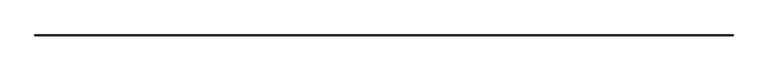
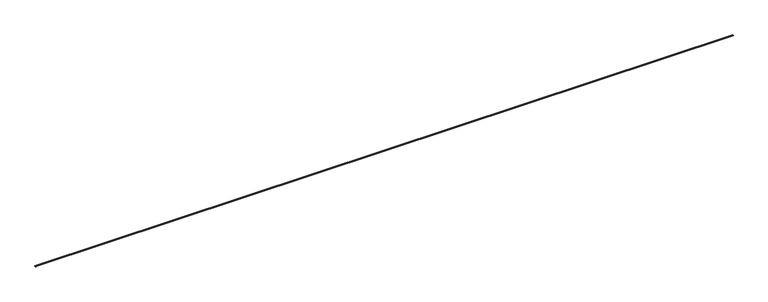
"""IFC4 building model written with IfcOpenShell, lengths in millimetres: proxy geometry, Generic Models 3:Generic Models 1:4:Generic Models 1:4 : Generic Models 3:Generic Models 1:300625:1:Generic Models 1:4:Generic Models 1:4 : Generic Models 3:Generic Models 1:300625:1 : Generic Models 3:Generic Models 1:4:Generic Models 1:4 : Generic Models 3:Generic Models 1:300625:338780:2 : Generic Models 3:Generic Models 1:4:Generic Models 1:4 : Generic Models 3:Generic Models 1:300625:1:Generic Models 1:4:Generic Models 1:4 : Generic Models 3:Generic Models 1:300625:1 : Generic Models 3:Generic Models 1:4:Generic Models 1:4 : Generic Models 3:Generic Models 1:300625:338780:317135."""

import ifcopenshell
import ifcopenshell.guid

model = None  # the IFC model being written
_history = None  # IfcOwnerHistory: only IFC2X3 demands one
_inside = {}  # id of a spatial element -> (the spatial element, [elements in it])
_under = {}  # id of a project, library or spatial element -> (it, [spatial elements below it])
_declared = {}  # id of a project -> (the project, [libraries it declares])
_typed = {}  # id of a type object -> (the type object, [elements of that type])
_made_of = {}  # id of a material, layer set ... -> (it, [elements and type objects made of it])


def new_model(schema):
    """Start an empty IFC model of exactly this schema.

    Asked for "IFC4X3", IfcOpenShell would pick the latest addendum, in which some entities
    have other attributes; the version numbers below select the first issue.
    IFC2X3 requires an IfcOwnerHistory on every rooted entity: one is made here for all.
    """
    global model, _history
    if schema == "IFC4X3":
        model = ifcopenshell.file(schema_version=(4, 3, 0, 0))
    else:
        model = ifcopenshell.file(schema=schema)
    _inside.clear()
    _under.clear()
    _declared.clear()
    _typed.clear()
    _made_of.clear()
    _history = None
    if model.schema == "IFC2X3":
        org = make("IfcOrganization", Name="unknown")
        user = make(
            "IfcPersonAndOrganization",
            ThePerson=make("IfcPerson", FamilyName="unknown"),
            TheOrganization=org,
        )
        app = make(
            "IfcApplication",
            ApplicationDeveloper=org,
            Version="unknown",
            ApplicationFullName="unknown",
            ApplicationIdentifier="unknown",
        )
        _history = make(
            "IfcOwnerHistory",
            OwningUser=user,
            OwningApplication=app,
            ChangeAction="ADDED",
            CreationDate=0,
        )
    return model


def make(cls, **values):
    """One entity of the class cls with the attributes given. An attribute that is None is left unset."""
    return model.create_entity(
        cls, **{name: value for name, value in values.items() if value is not None}
    )


def rooted(cls, **values):
    """An entity with a GlobalId (a new one), such as an element, a storey or a relation."""
    return make(cls, GlobalId=ifcopenshell.guid.new(), OwnerHistory=_history, **values)


def si_unit(unit_type, name, prefix=None):
    """IfcSIUnit, for example si_unit("LENGTHUNIT", "METRE", prefix="MILLI")."""
    return make("IfcSIUnit", UnitType=unit_type, Prefix=prefix, Name=name)


def assignment(units):
    """IfcUnitAssignment: the units of a project."""
    return None if units is None else make("IfcUnitAssignment", Units=units)


def point(xyz):
    """IfcCartesianPoint."""
    return None if xyz is None else make("IfcCartesianPoint", Coordinates=xyz)


def direction(xyz):
    """IfcDirection."""
    return None if xyz is None else make("IfcDirection", DirectionRatios=xyz)


def frame(location, z_axis=None, x_axis=None):
    """IfcAxis2Placement3D, a coordinate frame: its origin and axes. An axis left out is left unset."""
    return make(
        "IfcAxis2Placement3D",
        Location=point(location),
        Axis=direction(z_axis),
        RefDirection=direction(x_axis),
    )


def origin():
    """The frame at (0, 0, 0) with its axes left unset."""
    return frame((0.0, 0.0, 0.0))


def place(relative_to, where):
    """IfcLocalPlacement: puts the frame where relative to a parent placement (None: the world)."""
    return make(
        "IfcLocalPlacement", PlacementRelTo=relative_to, RelativePlacement=where
    )


def context(
    kind, dimensions, precision=None, world=None, true_north=None, identifier=None
):
    """IfcGeometricRepresentationContext, for example the 3D "Model" context."""
    return make(
        "IfcGeometricRepresentationContext",
        ContextIdentifier=identifier,
        ContextType=kind,
        CoordinateSpaceDimension=dimensions,
        Precision=precision,
        WorldCoordinateSystem=world,
        TrueNorth=true_north,
    )


def project(units=None, contexts=None):
    """IfcProject with its units and contexts."""
    return rooted(
        "IfcProject",
        Name="project",
        RepresentationContexts=contexts,
        UnitsInContext=assignment(units),
    )


def spatial(cls, under=None, at=None, **own):
    """A site, building, storey or space (cls), placed at a placement, below another one or the project."""
    s = rooted(cls, ObjectPlacement=at, **own)
    if under is not None:
        _under.setdefault(under.id(), (under, []))[1].append(s)
    return s


def polyline(points):
    """IfcPolyline through the points."""
    return make("IfcPolyline", Points=[point(p) for p in points])


def outline(outer, holes=None, kind="AREA"):
    """IfcArbitraryClosedProfileDef: a profile drawn as a closed curve; with holes, ...WithVoids."""
    if holes is None:
        return make("IfcArbitraryClosedProfileDef", ProfileType=kind, OuterCurve=outer)
    return make(
        "IfcArbitraryProfileDefWithVoids",
        ProfileType=kind,
        OuterCurve=outer,
        InnerCurves=holes,
    )


def extrude(swept, where, along, depth):
    """IfcExtrudedAreaSolid: the profile swept, set in the frame where, extruded along a direction by depth."""
    return make(
        "IfcExtrudedAreaSolid",
        SweptArea=swept,
        Position=where,
        ExtrudedDirection=direction(along),
        Depth=depth,
    )


def shape(context_of_items, identifier, shape_type, items):
    """IfcShapeRepresentation: the items that make up one representation, for example the "Body"."""
    return make(
        "IfcShapeRepresentation",
        ContextOfItems=context_of_items,
        RepresentationIdentifier=identifier,
        RepresentationType=shape_type,
        Items=items,
    )


def source(mapping_origin, context_of_items, identifier, shape_type, items):
    """IfcRepresentationMap: a shape defined once, which mapped items show again and again."""
    return make(
        "IfcRepresentationMap",
        MappingOrigin=mapping_origin,
        MappedRepresentation=shape(context_of_items, identifier, shape_type, items),
    )


def transform(
    local_origin,
    x_axis=None,
    y_axis=None,
    z_axis=None,
    scale=None,
    scale2=None,
    scale3=None,
    uniform=True,
):
    """IfcCartesianTransformationOperator3D, or its non-uniform kind. x_axis, y_axis, z_axis: its Axis1, 2, 3."""
    if uniform:
        return make(
            "IfcCartesianTransformationOperator3D",
            Axis1=direction(x_axis),
            Axis2=direction(y_axis),
            LocalOrigin=point(local_origin),
            Scale=scale,
            Axis3=direction(z_axis),
        )
    return make(
        "IfcCartesianTransformationOperator3DnonUniform",
        Axis1=direction(x_axis),
        Axis2=direction(y_axis),
        LocalOrigin=point(local_origin),
        Scale=scale,
        Axis3=direction(z_axis),
        Scale2=scale2,
        Scale3=scale3,
    )


def mapped(mapping_source, mapping_target):
    """IfcMappedItem: shows the shape of a source again, moved by a transform."""
    return make(
        "IfcMappedItem", MappingSource=mapping_source, MappingTarget=mapping_target
    )


def made_of(thing, what):
    """Note that an element or type object is made of a material, layer set ...; save() writes the relation."""
    if what is not None:
        _made_of.setdefault(what.id(), (what, []))[1].append(thing)
    return thing


def element(
    cls,
    number,
    at=None,
    inside=None,
    cuts=None,
    type_object=None,
    material=None,
    context=None,
    identifier="Body",
    shape_type=None,
    held_by="IfcProductDefinitionShape",
    body=None,
    shapes=None,
    **own,
):
    """One element of the class cls, such as IfcWall. Its Tag is "e" and its number.

    at: its placement. inside: the storey or other place that contains it. cuts: it is an
    opening in that element (IfcRelVoidsElement). A single representation is given by context,
    identifier, shape_type and body (its items); several are given by shapes. held_by: the class
    of the entity that holds the representations. save() writes the other relations.
    """
    e = rooted(cls, Tag="e%d" % number, ObjectPlacement=at, **own)
    if body is not None:
        shapes = [shape(context, identifier, shape_type, body)]
    if shapes is not None:
        e.Representation = make(held_by, Representations=shapes)
    if inside is not None:
        _inside.setdefault(inside.id(), (inside, []))[1].append(e)
    if cuts is not None:
        rooted(
            "IfcRelVoidsElement", RelatingBuildingElement=cuts, RelatedOpeningElement=e
        )
    if type_object is not None:
        _typed.setdefault(type_object.id(), (type_object, []))[1].append(e)
    return made_of(e, material)


def aggregate(whole, parts):
    """IfcRelAggregates: a whole, such as a stair, and the parts it consists of."""
    return rooted("IfcRelAggregates", RelatingObject=whole, RelatedObjects=parts)


def save(model, path):
    """Write the relations noted so far, then the file.

    IfcRelAggregates (storeys below a building ...), IfcRelContainedInSpatialStructure (elements
    in a storey), IfcRelDefinesByType, IfcRelAssociatesMaterial and IfcRelDeclares: one each for
    every whole, place, type object, material and project.
    """
    for whole, parts in _under.values():
        aggregate(whole, parts)
    for where, things in _inside.values():
        rooted(
            "IfcRelContainedInSpatialStructure",
            RelatedElements=things,
            RelatingStructure=where,
        )
    for kind, things in _typed.values():
        rooted("IfcRelDefinesByType", RelatedObjects=things, RelatingType=kind)
    for what, things in _made_of.values():
        rooted("IfcRelAssociatesMaterial", RelatedObjects=things, RelatingMaterial=what)
    for by, libraries in _declared.values():
        rooted("IfcRelDeclares", RelatingContext=by, RelatedDefinitions=libraries)
    model.write(path)


def generic_models_aa0125ff(model_context):
    return source(origin(), model_context, "Body", "SweptSolid", [
        extrude(outline(polyline([(-579088.4739295, 3713.8232545), (-579094.6612723, 3713.8232545), (-579094.1146795, 3714.4746585), (-579093.8638533, 3715.4107545), (-579094.1146795, 3716.3468505), (-579094.6612723, 3716.9982545), (-579088.4739295, 3716.9982545), (-579089.0205223, 3716.3468505), (-579089.2713485, 3715.4107545), (-579089.0205223, 3714.4746585), (-579088.4739295, 3713.8232545)])), frame((591306.0367239, 0.0, 0.0), z_axis=(1.0, 0.0, 0.0), x_axis=(0.0, 1.0, 0.0)), (0.0, 0.0, 1.0), 4876.8),
    ])


if __name__ == "__main__":
    model = new_model("IFC4")
    model_context = context("Model", 3, world=origin())
    ifc_project = project(units=[si_unit("LENGTHUNIT", "METRE", prefix="MILLI")], contexts=[model_context])
    site = spatial("IfcSite", under=ifc_project)
    building = spatial("IfcBuilding", under=site)
    placement = place(None, origin())
    generic_models_shape = generic_models_aa0125ff(model_context)
    element("IfcBuildingElementProxy", 1, Name="Generic Models 3:Generic Models 1:4:Generic Models 1:4 : Generic Models 3:Generic Models 1:300625:1:Generic Models 1:4:Generic Models 1:4 : Generic Models 3:Generic Models 1:300625:1 : Generic Models 3:Generic Models 1:4:Generic Models 1:4 : Generic Models 3:Generic Models 1:300625:338780:2 : Generic Models 3:Generic Models 1:4:Generic Models 1:4 : Generic Models 3:Generic Models 1:300625:1:Generic Models 1:4:Generic Models 1:4 : Generic Models 3:Generic Models 1:300625:1 : Generic Models 3:Generic Models 1:4:Generic Models 1:4 : Generic Models 3:Generic Models 1:300625:338780:317135", ObjectType="Generic Models 3:Generic Models 1:4:Generic Models 1:4 : Generic Models 3:Generic Models 1:300625:1:Generic Models 1:4:Generic Models 1:4 : Generic Models 3:Generic Models 1:300625:1 : Generic Models 3:Generic Models 1:4:Generic Models 1:4 : Generic Models 3:Generic Models 1:300625:338780:2 : Generic Models 3:Generic Models 1:4:Generic Models 1:4 : Generic Models 3:Generic Models 1:300625:1:Generic Models 1:4:Generic Models 1:4 : Generic Models 3:Generic Models 1:300625:1 : Generic Models 3:Generic Models 1:4:Generic Models 1:4 : Generic Models 3:Generic Models 1:300625:338780:317135", at=placement, inside=building, context=model_context, shape_type="MappedRepresentation", body=[
        mapped(generic_models_shape, transform((0.0, 0.0, 0.0), x_axis=(1.0, 0.0, 0.0), y_axis=(0.0, 1.0, 0.0), z_axis=(0.0, 0.0, 1.0))),
    ])
    save(model, "model.ifc")

# Revit data of these elements
# Type "Generic Models 3:Generic Models 1:4:Generic Models 1:4 : Generic Models 3:Generic Models 1:300625:1:Generic Models 1:4:Generic Models 1:4 : Generic Models 3:Generic Models 1:300625:1 : Generic Models 3:Generic Models 1:4:Generic Models 1:4 : Generic Models 3:Generic Models 1:300625:338780:2 : Generic Models 3:Generic Models 1:4:Generic Models 1:4 : Generic Models 3:Generic Models 1:300625:1:Generic Models 1:4:Generic Models 1:4 : Generic Models 3:Generic Models 1:300625:1 : Generic Models 3:Generic Models 1:4:Generic Models 1:4 : Generic Models 3:Generic Models 1:300625:338780:317135"
#   NameOverride = "Generic Models 3:Generic Models 1:4:Generic Models 1:4 : Generic Models 3:Generic Models 1:300625:1:Generic Models 1:4:Generic Models 1:4 : Generic Models 3:Generic Models 1:300625:1 : Generic Models 3:Generic Models 1:4:Generic Models 1:4 : Generic Models 3:Generic Models 1:300625:338780:317135"
#   ObjectTypeOverride = "Generic Models 1:4:Generic Models 1:4 : Generic Models 3:Generic Models 1:300625:1 : Generic Models 3:Generic Models 1:4:Generic Models 1:4 : Generic Models 3:Generic Models 1:300625:338780"
#   Reference = "Generic Models 1"
#   Tag = "317135"
# Element 1 (IfcBuildingElementProxy, "Generic Models 3:Generic Models 1:4:Generic Models 1:4 : Generic Models 3:Generic Models 1:300625:1:Generic Models 1:4:Generic Models 1:4 : Generic Models 3:Generic Models 1:300625:1 : Generic Models 3:Generic Models 1:4:Generic Models 1:4 : Generic Models 3:Generic Models 1:300625:338780:2 : Generic Models 3:Generic Models 1:4:Generic Models 1:4 : Generic Models 3:Generic Models 1:300625:1:Generic Models 1:4:Generic Models 1:4 : Generic Models 3:Generic Models 1:300625:1 : Generic Models 3:Generic Models 1:4:Generic Models 1:4 : Generic Models 3:Generic Models 1:300625:338780:317135")
#   Materials on its faces: "SEALANT & BACKER ROD"
# Materials
#   "SEALANT & BACKER ROD": class "Unassigned", colour RGB 120 120 120, transparency 0, Cost = 0
